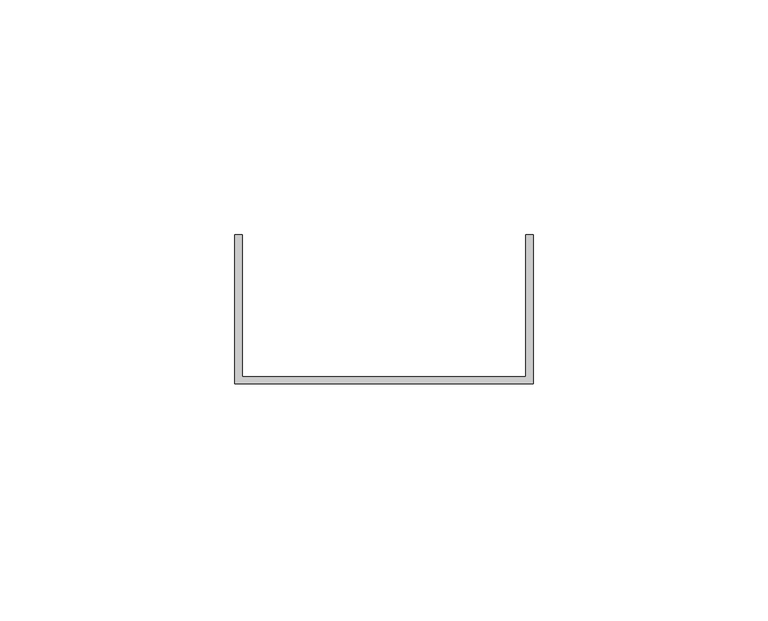
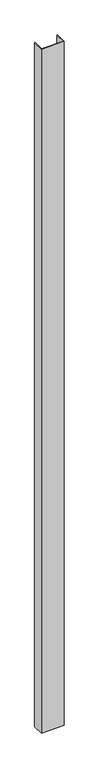
"""IFC4 building model written with IfcOpenShell, lengths in millimetres: proxy geometry, Generic Models 7:Generic Models 1:3:Generic Models 1:3 : Generic Models 7:Generic Models 1:305549:3:Generic Models 1:3:Generic Models 1:3 : Generic Models 7:Generic Models 1:305549:3 : Generic Models 7:Generic Models 1:3:Generic Models 1:3 : Generic Models 7:Generic Models 1:305549:301244:27 : Generic Models 7:Generic Models 1:3:Generic Models 1:3 : Generic Models 7:Generic Models 1:305549:3:Generic Models 1:3:Generic Models 1:3 : Generic Models 7:Generic Models 1:305549:3 : Generic Models 7:Generic Models 1:3:Generic Models 1:3 : Generic Models 7:Generic Models 1:305549:301244:308848."""

from ifc_helpers import new_model, si_unit, frame, origin, place, context, project, spatial, polyline, outline, extrude, source, transform, mapped, element, save


def generic_models_97e3ebf6(model_context):
    return source(origin(), model_context, "Body", "SweptSolid", [
        extrude(outline(polyline([(560340.2617239, -572587.1913841), (560276.7617239, -572587.1913841), (560276.7617239, -572555.4413841), (560278.3492239, -572555.4413841), (560278.3492239, -572585.6038841), (560338.6742239, -572585.6038841), (560338.6742239, -572555.4413841), (560340.2617239, -572555.4413841), (560340.2617239, -572587.1913841)])), frame((0.0, 0.0, 4133.81326), z_axis=(0.0, 0.0, 1.0), x_axis=(1.0, 0.0, 0.0)), (0.0, 0.0, 1.0), 2000.28674),
    ])


if __name__ == "__main__":
    model = new_model("IFC4")
    model_context = context("Model", 3, world=origin())
    ifc_project = project(units=[si_unit("LENGTHUNIT", "METRE", prefix="MILLI")], contexts=[model_context])
    site = spatial("IfcSite", under=ifc_project)
    building = spatial("IfcBuilding", under=site)
    placement = place(None, origin())
    generic_models_shape = generic_models_97e3ebf6(model_context)
    element("IfcBuildingElementProxy", 1, Name="Generic Models 7:Generic Models 1:3:Generic Models 1:3 : Generic Models 7:Generic Models 1:305549:3:Generic Models 1:3:Generic Models 1:3 : Generic Models 7:Generic Models 1:305549:3 : Generic Models 7:Generic Models 1:3:Generic Models 1:3 : Generic Models 7:Generic Models 1:305549:301244:27 : Generic Models 7:Generic Models 1:3:Generic Models 1:3 : Generic Models 7:Generic Models 1:305549:3:Generic Models 1:3:Generic Models 1:3 : Generic Models 7:Generic Models 1:305549:3 : Generic Models 7:Generic Models 1:3:Generic Models 1:3 : Generic Models 7:Generic Models 1:305549:301244:308848", ObjectType="Generic Models 7:Generic Models 1:3:Generic Models 1:3 : Generic Models 7:Generic Models 1:305549:3:Generic Models 1:3:Generic Models 1:3 : Generic Models 7:Generic Models 1:305549:3 : Generic Models 7:Generic Models 1:3:Generic Models 1:3 : Generic Models 7:Generic Models 1:305549:301244:27 : Generic Models 7:Generic Models 1:3:Generic Models 1:3 : Generic Models 7:Generic Models 1:305549:3:Generic Models 1:3:Generic Models 1:3 : Generic Models 7:Generic Models 1:305549:3 : Generic Models 7:Generic Models 1:3:Generic Models 1:3 : Generic Models 7:Generic Models 1:305549:301244:308848", at=placement, inside=building, context=model_context, shape_type="MappedRepresentation", body=[
        mapped(generic_models_shape, transform((0.0, 0.0, 0.0), x_axis=(1.0, 0.0, 0.0), y_axis=(0.0, 1.0, 0.0), z_axis=(0.0, 0.0, 1.0))),
    ])
    save(model, "model.ifc")

# Revit data of these elements
# Type "Generic Models 7:Generic Models 1:3:Generic Models 1:3 : Generic Models 7:Generic Models 1:305549:3:Generic Models 1:3:Generic Models 1:3 : Generic Models 7:Generic Models 1:305549:3 : Generic Models 7:Generic Models 1:3:Generic Models 1:3 : Generic Models 7:Generic Models 1:305549:301244:27 : Generic Models 7:Generic Models 1:3:Generic Models 1:3 : Generic Models 7:Generic Models 1:305549:3:Generic Models 1:3:Generic Models 1:3 : Generic Models 7:Generic Models 1:305549:3 : Generic Models 7:Generic Models 1:3:Generic Models 1:3 : Generic Models 7:Generic Models 1:305549:301244:308848"
#   NameOverride = "Generic Models 7:Generic Models 1:3:Generic Models 1:3 : Generic Models 7:Generic Models 1:305549:3:Generic Models 1:3:Generic Models 1:3 : Generic Models 7:Generic Models 1:305549:3 : Generic Models 7:Generic Models 1:3:Generic Models 1:3 : Generic Models 7:Generic Models 1:305549:301244:308848"
#   ObjectTypeOverride = "Generic Models 1:3:Generic Models 1:3 : Generic Models 7:Generic Models 1:305549:3 : Generic Models 7:Generic Models 1:3:Generic Models 1:3 : Generic Models 7:Generic Models 1:305549:301244"
#   Reference = "Generic Models 1"
#   Tag = "308848"
# Element 1 (IfcBuildingElementProxy, "Generic Models 7:Generic Models 1:3:Generic Models 1:3 : Generic Models 7:Generic Models 1:305549:3:Generic Models 1:3:Generic Models 1:3 : Generic Models 7:Generic Models 1:305549:3 : Generic Models 7:Generic Models 1:3:Generic Models 1:3 : Generic Models 7:Generic Models 1:305549:301244:27 : Generic Models 7:Generic Models 1:3:Generic Models 1:3 : Generic Models 7:Generic Models 1:305549:3:Generic Models 1:3:Generic Models 1:3 : Generic Models 7:Generic Models 1:305549:3 : Generic Models 7:Generic Models 1:3:Generic Models 1:3 : Generic Models 7:Generic Models 1:305549:301244:308848")
#   Materials on its faces: "GALVANIZED U-CHANNEL (250T125-33)"
# Materials
#   "GALVANIZED U-CHANNEL (250T125-33)": class "Unassigned", colour RGB 202 201 200, transparency 0, Keynote = "M05451300.02", Cost = 0
